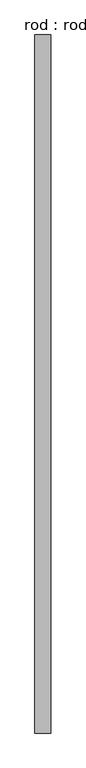
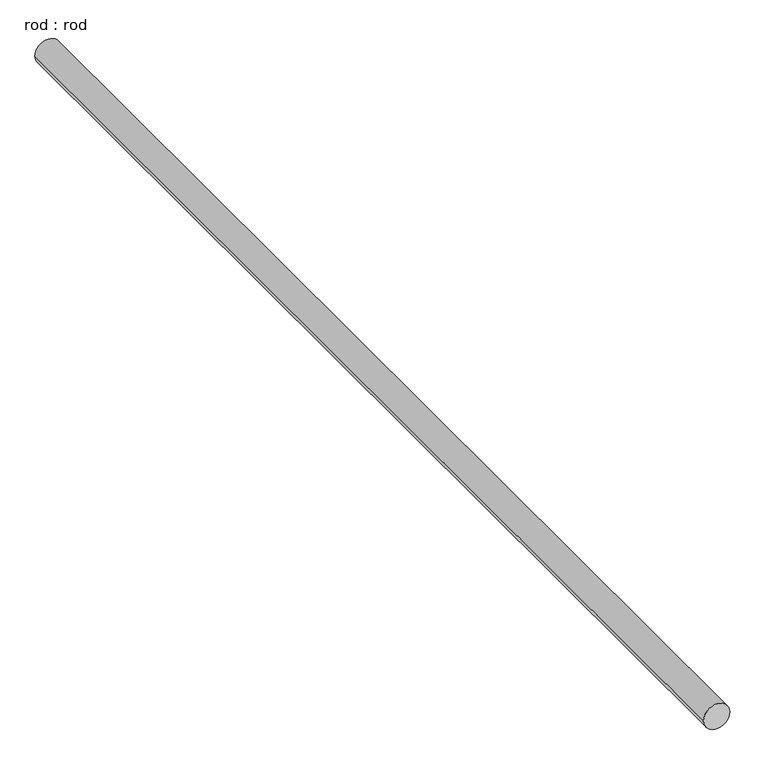
"""IFC4 building model written with IfcOpenShell, lengths in millimetres: proxy geometry, rod : rod."""

from ifc_helpers import new_model, si_unit, point, frame, frame_2d, origin, place, context, project, spatial, circle_curve, trimmed, segment, composite_curve, outline, extrude, source, transform, mapped, element, save


def rod_rod_d3eb37dc(model_context):
    return source(origin(), model_context, "Body", "SweptSolid", [
        extrude(outline(composite_curve([segment(trimmed(circle_curve(frame_2d((0.0108462, 0.0)), 200.0), [point((0.0108462, 200.0))], [point((0.0108462, -200.0))], False, "CARTESIAN"), True, "CONTINUOUS"), segment(trimmed(circle_curve(frame_2d((0.0108462, 0.0)), 200.0), [point((0.0108462, -200.0))], [point((0.0108462, 200.0))], False, "CARTESIAN"), True, "CONTINUOUS")], self_intersect=False)), frame((0.0, -4733.1642418, 0.0), z_axis=(0.0, 1.0, 0.0), x_axis=(0.0, 0.0, 1.0)), (0.0, 0.0, 1.0), 17651.7857143),
    ])


if __name__ == "__main__":
    model = new_model("IFC4")
    model_context = context("Model", 3, world=origin())
    ifc_project = project(units=[si_unit("LENGTHUNIT", "METRE", prefix="MILLI")], contexts=[model_context])
    site = spatial("IfcSite", under=ifc_project)
    building = spatial("IfcBuilding", under=site)
    placement = place(None, origin())
    rod_rod_shape = rod_rod_d3eb37dc(model_context)
    element("IfcBuildingElementProxy", 1, Name="rod : rod", ObjectType="rod : rod", at=placement, inside=building, context=model_context, shape_type="MappedRepresentation", body=[
        mapped(rod_rod_shape, transform((0.0, 0.0, 0.0), x_axis=(1.0, 0.0, 0.0), y_axis=(0.0, 1.0, 0.0), z_axis=(0.0, 0.0, 1.0))),
    ])
    save(model, "model.ifc")

# Revit data of these elements
# Type "rod : rod"
#   Default Elevation = 0
